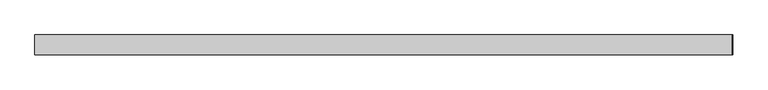
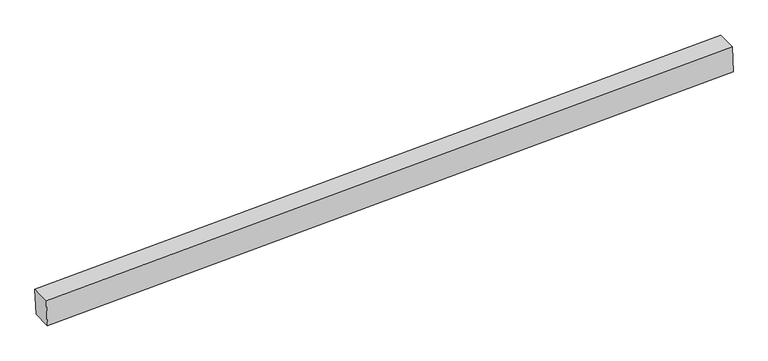
"""IFC4 building model written with IfcOpenShell, lengths in millimetres: proxy geometry, Generic Models 7:Generic Models 1:8:Generic Models 1:8 : Generic Models 7:Generic Models 1:337419:30 : Generic Models 7:Generic Models 1:8:Generic Models 1:8 : Generic Models 7:Generic Models 1:337419:315935."""

import ifcopenshell
import ifcopenshell.guid

model = None  # the IFC model being written
_history = None  # IfcOwnerHistory: only IFC2X3 demands one
_inside = {}  # id of a spatial element -> (the spatial element, [elements in it])
_under = {}  # id of a project, library or spatial element -> (it, [spatial elements below it])
_declared = {}  # id of a project -> (the project, [libraries it declares])
_typed = {}  # id of a type object -> (the type object, [elements of that type])
_made_of = {}  # id of a material, layer set ... -> (it, [elements and type objects made of it])


def new_model(schema):
    """Start an empty IFC model of exactly this schema.

    Asked for "IFC4X3", IfcOpenShell would pick the latest addendum, in which some entities
    have other attributes; the version numbers below select the first issue.
    IFC2X3 requires an IfcOwnerHistory on every rooted entity: one is made here for all.
    """
    global model, _history
    if schema == "IFC4X3":
        model = ifcopenshell.file(schema_version=(4, 3, 0, 0))
    else:
        model = ifcopenshell.file(schema=schema)
    _inside.clear()
    _under.clear()
    _declared.clear()
    _typed.clear()
    _made_of.clear()
    _history = None
    if model.schema == "IFC2X3":
        org = make("IfcOrganization", Name="unknown")
        user = make(
            "IfcPersonAndOrganization",
            ThePerson=make("IfcPerson", FamilyName="unknown"),
            TheOrganization=org,
        )
        app = make(
            "IfcApplication",
            ApplicationDeveloper=org,
            Version="unknown",
            ApplicationFullName="unknown",
            ApplicationIdentifier="unknown",
        )
        _history = make(
            "IfcOwnerHistory",
            OwningUser=user,
            OwningApplication=app,
            ChangeAction="ADDED",
            CreationDate=0,
        )
    return model


def make(cls, **values):
    """One entity of the class cls with the attributes given. An attribute that is None is left unset."""
    return model.create_entity(
        cls, **{name: value for name, value in values.items() if value is not None}
    )


def rooted(cls, **values):
    """An entity with a GlobalId (a new one), such as an element, a storey or a relation."""
    return make(cls, GlobalId=ifcopenshell.guid.new(), OwnerHistory=_history, **values)


def si_unit(unit_type, name, prefix=None):
    """IfcSIUnit, for example si_unit("LENGTHUNIT", "METRE", prefix="MILLI")."""
    return make("IfcSIUnit", UnitType=unit_type, Prefix=prefix, Name=name)


def assignment(units):
    """IfcUnitAssignment: the units of a project."""
    return None if units is None else make("IfcUnitAssignment", Units=units)


def point(xyz):
    """IfcCartesianPoint."""
    return None if xyz is None else make("IfcCartesianPoint", Coordinates=xyz)


def direction(xyz):
    """IfcDirection."""
    return None if xyz is None else make("IfcDirection", DirectionRatios=xyz)


def frame(location, z_axis=None, x_axis=None):
    """IfcAxis2Placement3D, a coordinate frame: its origin and axes. An axis left out is left unset."""
    return make(
        "IfcAxis2Placement3D",
        Location=point(location),
        Axis=direction(z_axis),
        RefDirection=direction(x_axis),
    )


def origin():
    """The frame at (0, 0, 0) with its axes left unset."""
    return frame((0.0, 0.0, 0.0))


def place(relative_to, where):
    """IfcLocalPlacement: puts the frame where relative to a parent placement (None: the world)."""
    return make(
        "IfcLocalPlacement", PlacementRelTo=relative_to, RelativePlacement=where
    )


def context(
    kind, dimensions, precision=None, world=None, true_north=None, identifier=None
):
    """IfcGeometricRepresentationContext, for example the 3D "Model" context."""
    return make(
        "IfcGeometricRepresentationContext",
        ContextIdentifier=identifier,
        ContextType=kind,
        CoordinateSpaceDimension=dimensions,
        Precision=precision,
        WorldCoordinateSystem=world,
        TrueNorth=true_north,
    )


def project(units=None, contexts=None):
    """IfcProject with its units and contexts."""
    return rooted(
        "IfcProject",
        Name="project",
        RepresentationContexts=contexts,
        UnitsInContext=assignment(units),
    )


def spatial(cls, under=None, at=None, **own):
    """A site, building, storey or space (cls), placed at a placement, below another one or the project."""
    s = rooted(cls, ObjectPlacement=at, **own)
    if under is not None:
        _under.setdefault(under.id(), (under, []))[1].append(s)
    return s


def polyline(points):
    """IfcPolyline through the points."""
    return make("IfcPolyline", Points=[point(p) for p in points])


def outline(outer, holes=None, kind="AREA"):
    """IfcArbitraryClosedProfileDef: a profile drawn as a closed curve; with holes, ...WithVoids."""
    if holes is None:
        return make("IfcArbitraryClosedProfileDef", ProfileType=kind, OuterCurve=outer)
    return make(
        "IfcArbitraryProfileDefWithVoids",
        ProfileType=kind,
        OuterCurve=outer,
        InnerCurves=holes,
    )


def extrude(swept, where, along, depth):
    """IfcExtrudedAreaSolid: the profile swept, set in the frame where, extruded along a direction by depth."""
    return make(
        "IfcExtrudedAreaSolid",
        SweptArea=swept,
        Position=where,
        ExtrudedDirection=direction(along),
        Depth=depth,
    )


def shape(context_of_items, identifier, shape_type, items):
    """IfcShapeRepresentation: the items that make up one representation, for example the "Body"."""
    return make(
        "IfcShapeRepresentation",
        ContextOfItems=context_of_items,
        RepresentationIdentifier=identifier,
        RepresentationType=shape_type,
        Items=items,
    )


def source(mapping_origin, context_of_items, identifier, shape_type, items):
    """IfcRepresentationMap: a shape defined once, which mapped items show again and again."""
    return make(
        "IfcRepresentationMap",
        MappingOrigin=mapping_origin,
        MappedRepresentation=shape(context_of_items, identifier, shape_type, items),
    )


def transform(
    local_origin,
    x_axis=None,
    y_axis=None,
    z_axis=None,
    scale=None,
    scale2=None,
    scale3=None,
    uniform=True,
):
    """IfcCartesianTransformationOperator3D, or its non-uniform kind. x_axis, y_axis, z_axis: its Axis1, 2, 3."""
    if uniform:
        return make(
            "IfcCartesianTransformationOperator3D",
            Axis1=direction(x_axis),
            Axis2=direction(y_axis),
            LocalOrigin=point(local_origin),
            Scale=scale,
            Axis3=direction(z_axis),
        )
    return make(
        "IfcCartesianTransformationOperator3DnonUniform",
        Axis1=direction(x_axis),
        Axis2=direction(y_axis),
        LocalOrigin=point(local_origin),
        Scale=scale,
        Axis3=direction(z_axis),
        Scale2=scale2,
        Scale3=scale3,
    )


def mapped(mapping_source, mapping_target):
    """IfcMappedItem: shows the shape of a source again, moved by a transform."""
    return make(
        "IfcMappedItem", MappingSource=mapping_source, MappingTarget=mapping_target
    )


def made_of(thing, what):
    """Note that an element or type object is made of a material, layer set ...; save() writes the relation."""
    if what is not None:
        _made_of.setdefault(what.id(), (what, []))[1].append(thing)
    return thing


def element(
    cls,
    number,
    at=None,
    inside=None,
    cuts=None,
    type_object=None,
    material=None,
    context=None,
    identifier="Body",
    shape_type=None,
    held_by="IfcProductDefinitionShape",
    body=None,
    shapes=None,
    **own,
):
    """One element of the class cls, such as IfcWall. Its Tag is "e" and its number.

    at: its placement. inside: the storey or other place that contains it. cuts: it is an
    opening in that element (IfcRelVoidsElement). A single representation is given by context,
    identifier, shape_type and body (its items); several are given by shapes. held_by: the class
    of the entity that holds the representations. save() writes the other relations.
    """
    e = rooted(cls, Tag="e%d" % number, ObjectPlacement=at, **own)
    if body is not None:
        shapes = [shape(context, identifier, shape_type, body)]
    if shapes is not None:
        e.Representation = make(held_by, Representations=shapes)
    if inside is not None:
        _inside.setdefault(inside.id(), (inside, []))[1].append(e)
    if cuts is not None:
        rooted(
            "IfcRelVoidsElement", RelatingBuildingElement=cuts, RelatedOpeningElement=e
        )
    if type_object is not None:
        _typed.setdefault(type_object.id(), (type_object, []))[1].append(e)
    return made_of(e, material)


def aggregate(whole, parts):
    """IfcRelAggregates: a whole, such as a stair, and the parts it consists of."""
    return rooted("IfcRelAggregates", RelatingObject=whole, RelatedObjects=parts)


def save(model, path):
    """Write the relations noted so far, then the file.

    IfcRelAggregates (storeys below a building ...), IfcRelContainedInSpatialStructure (elements
    in a storey), IfcRelDefinesByType, IfcRelAssociatesMaterial and IfcRelDeclares: one each for
    every whole, place, type object, material and project.
    """
    for whole, parts in _under.values():
        aggregate(whole, parts)
    for where, things in _inside.values():
        rooted(
            "IfcRelContainedInSpatialStructure",
            RelatedElements=things,
            RelatingStructure=where,
        )
    for kind, things in _typed.values():
        rooted("IfcRelDefinesByType", RelatedObjects=things, RelatingType=kind)
    for what, things in _made_of.values():
        rooted("IfcRelAssociatesMaterial", RelatedObjects=things, RelatingMaterial=what)
    for by, libraries in _declared.values():
        rooted("IfcRelDeclares", RelatingContext=by, RelatedDefinitions=libraries)
    model.write(path)


def generic_models_890d81a9(model_context):
    return source(origin(), model_context, "Body", "SweptSolid", [
        extrude(outline(polyline([(3818.9012888, 558136.9256261), (3628.5664384, 558144.8562449), (3831.5897382, 563017.4154421), (4021.9397427, 563009.8485204), (3818.9012888, 558136.9256261)])), frame((0.0, -577565.5913841, 0.0), z_axis=(0.0, 1.0, 0.0), x_axis=(0.0, 0.0, 1.0)), (0.0, 0.0, 1.0), 139.7),
    ])


if __name__ == "__main__":
    model = new_model("IFC4")
    model_context = context("Model", 3, world=origin())
    ifc_project = project(units=[si_unit("LENGTHUNIT", "METRE", prefix="MILLI")], contexts=[model_context])
    site = spatial("IfcSite", under=ifc_project)
    building = spatial("IfcBuilding", under=site)
    placement = place(None, origin())
    generic_models_shape = generic_models_890d81a9(model_context)
    element("IfcBuildingElementProxy", 1, Name="Generic Models 7:Generic Models 1:8:Generic Models 1:8 : Generic Models 7:Generic Models 1:337419:30 : Generic Models 7:Generic Models 1:8:Generic Models 1:8 : Generic Models 7:Generic Models 1:337419:315935", ObjectType="Generic Models 7:Generic Models 1:8:Generic Models 1:8 : Generic Models 7:Generic Models 1:337419:30 : Generic Models 7:Generic Models 1:8:Generic Models 1:8 : Generic Models 7:Generic Models 1:337419:315935", at=placement, inside=building, context=model_context, shape_type="MappedRepresentation", body=[
        mapped(generic_models_shape, transform((0.0, 0.0, 0.0), x_axis=(1.0, 0.0, 0.0), y_axis=(0.0, 1.0, 0.0), z_axis=(0.0, 0.0, 1.0))),
    ])
    save(model, "model.ifc")

# Revit data of these elements
# Type "Generic Models 7:Generic Models 1:8:Generic Models 1:8 : Generic Models 7:Generic Models 1:337419:30 : Generic Models 7:Generic Models 1:8:Generic Models 1:8 : Generic Models 7:Generic Models 1:337419:315935"
#   NameOverride = "Generic Models 7:Generic Models 1:8:Generic Models 1:8 : Generic Models 7:Generic Models 1:337419:315935"
#   ObjectTypeOverride = "Generic Models 1:8 : Generic Models 7:Generic Models 1:337419"
#   Reference = "Generic Models 1"
#   Tag = "315935"
# Element 1 (IfcBuildingElementProxy, "Generic Models 7:Generic Models 1:8:Generic Models 1:8 : Generic Models 7:Generic Models 1:337419:30 : Generic Models 7:Generic Models 1:8:Generic Models 1:8 : Generic Models 7:Generic Models 1:337419:315935")
#   Materials on its faces: "5 1/2\" X 7 1/2\" EXTERIOR GRADE GLULAM BEAMS"
# Materials
#   "5 1/2\" X 7 1/2\" EXTERIOR GRADE GLULAM BEAMS": class "Wood", colour RGB 183 134 68, transparency 0, Keynote = "M06181300.01", Description = "Pinus Echinata", Cost = 0
